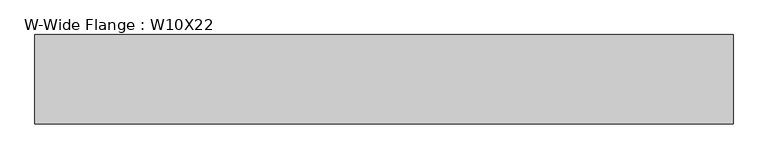
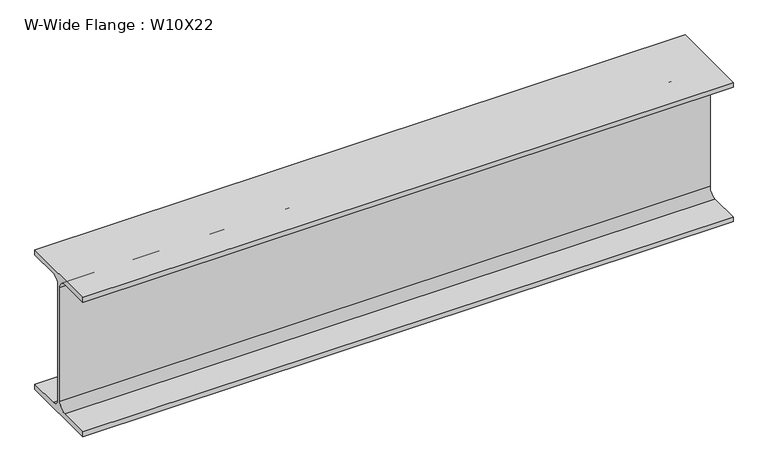
"""IFC4 building model written with IfcOpenShell, lengths in millimetres: beam geometry, W-Wide Flange : W10X22."""

from ifc_helpers import new_model, si_unit, point, frame, frame_2d, origin, place, context, project, spatial, polyline, circle_curve, trimmed, segment, composite_curve, outline, extrude, source, transform, mapped, element, save


def w_wide_flange_w10x22_69c26e3b(model_context):
    return source(origin(), model_context, "Body", "SweptSolid", [
        extrude(outline(composite_curve([segment(polyline([(73.025, -120.396), (73.025, -129.54), (-73.025, -129.54), (-73.025, -120.396), (-17.7165, -120.396)]), True, "CONTINUOUS"), segment(trimmed(circle_curve(frame_2d((-17.7165, -105.7275)), 14.6685), [point((-17.7165, -120.396))], [point((-3.048, -105.7275))], True, "CARTESIAN"), True, "CONTINUOUS"), segment(polyline([(-3.048, -105.7275), (-3.048, 105.7275)]), True, "CONTINUOUS"), segment(trimmed(circle_curve(frame_2d((-17.7165, 105.7275)), 14.6685), [point((-3.048, 105.7275))], [point((-17.7165, 120.396))], True, "CARTESIAN"), True, "CONTINUOUS"), segment(polyline([(-17.7165, 120.396), (-73.025, 120.396), (-73.025, 129.54), (73.025, 129.54), (73.025, 120.396), (17.7165, 120.396)]), True, "CONTINUOUS"), segment(trimmed(circle_curve(frame_2d((17.7165, 105.7275)), 14.6685), [point((17.7165, 120.396))], [point((3.048, 105.7275))], True, "CARTESIAN"), True, "CONTINUOUS"), segment(polyline([(3.048, 105.7275), (3.048, -105.7275)]), True, "CONTINUOUS"), segment(trimmed(circle_curve(frame_2d((17.7165, -105.7275)), 14.6685), [point((3.048, -105.7275))], [point((17.7165, -120.396))], True, "CARTESIAN"), True, "CONTINUOUS"), segment(polyline([(17.7165, -120.396), (73.025, -120.396)]), True, "CONTINUOUS")], self_intersect=False)), frame((-571.5, 0.0, 0.0), z_axis=(1.0, 0.0, 0.0), x_axis=(0.0, 1.0, 0.0)), (0.0, 0.0, 1.0), 1143.0),
    ])


if __name__ == "__main__":
    model = new_model("IFC4")
    model_context = context("Model", 3, world=origin())
    ifc_project = project(units=[si_unit("LENGTHUNIT", "METRE", prefix="MILLI")], contexts=[model_context])
    site = spatial("IfcSite", under=ifc_project)
    building = spatial("IfcBuilding", under=site)
    placement = place(None, origin())
    w_wide_flange_w10x22_shape = w_wide_flange_w10x22_69c26e3b(model_context)
    element("IfcBeam", 1, ObjectType="W-Wide Flange : W10X22", at=placement, inside=building, context=model_context, shape_type="MappedRepresentation", body=[
        mapped(w_wide_flange_w10x22_shape, transform((0.0, 0.0, 0.0), x_axis=(1.0, 0.0, 0.0), y_axis=(0.0, 1.0, 0.0), z_axis=(0.0, 0.0, 1.0))),
    ])
    save(model, "model.ifc")

# Revit data of these elements
# Type "W-Wide Flange : W10X22"
#   Assembly Code = "B10"
#   W = 22
#   Length [instance default] = 5' - 0"
#   bf = 0' - 5 3/4"
#   d = 0' - 10.2"
#   k = 0' - 0 15/16"
#   k2 = 0' - 0.5775"
#   tf = 0' - 0.36"
#   tw = 0' - 0.24"
#   A = 0.0450694 SF
#   Structural Material [instance default] = _STRUCTURAL STEEL (SEE STRUCT. DWGS)
# Element 1 (IfcBeam, "W-Wide Flange : W10X22")
#   Materials on its faces: "_STRUCTURAL STEEL (SEE STRUCT. DWGS)"
# Materials
#   "_STRUCTURAL STEEL (SEE STRUCT. DWGS)": class "Metal", colour RGB 199 199 199, transparency 0, Description = "Structural steel 50ksi", Cost = 0
